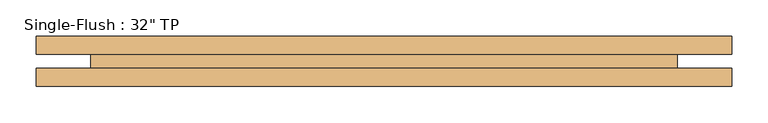
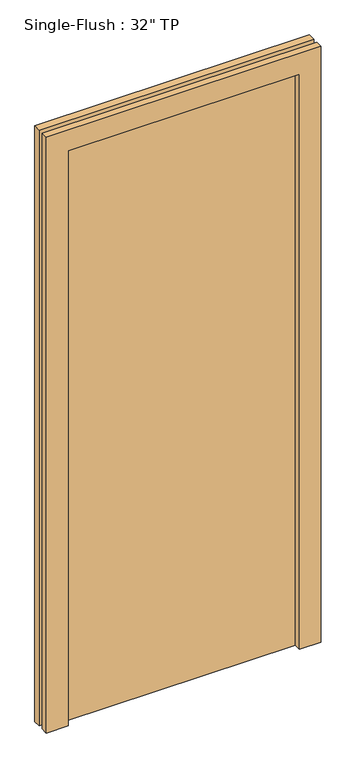
"""IFC4 building model written with IfcOpenShell, lengths in millimetres: door geometry."""

from ifc_helpers import new_model, si_unit, frame, origin, origin_with_axes, place, context, project, spatial, polyline, outline, extrude, source, transform, mapped, element, save


def door_1d070c31(model_context):
    return source(origin(), model_context, "Body", "SweptSolid", [
        extrude(outline(polyline([(2209.8, -482.6), (0.0, -482.6), (0.0, -406.4), (2133.6, -406.4), (2133.6, 406.4), (0.0, 406.4), (0.0, 482.6), (2209.8, 482.6), (2209.8, -482.6)])), frame((0.0, -34.925, 0.0), z_axis=(0.0, 1.0, 0.0), x_axis=(0.0, 0.0, 1.0)), (0.0, 0.0, 1.0), 25.4),
        extrude(outline(polyline([(2209.8, 482.6), (2209.8, -482.6), (0.0, -482.6), (0.0, -406.4), (2133.6, -406.4), (2133.6, 406.4), (0.0, 406.4), (0.0, 482.6), (2209.8, 482.6)])), frame((0.0, 9.525, 0.0), z_axis=(0.0, 1.0, 0.0), x_axis=(0.0, 0.0, 1.0)), (0.0, 0.0, 1.0), 25.4),
        extrude(outline(polyline([(406.4, 9.525), (406.4, -9.525), (-406.4, -9.525), (-406.4, 9.525), (406.4, 9.525)])), origin_with_axes(), (0.0, 0.0, 1.0), 2133.6),
    ])


if __name__ == "__main__":
    model = new_model("IFC4")
    model_context = context("Model", 3, world=origin())
    ifc_project = project(units=[si_unit("LENGTHUNIT", "METRE", prefix="MILLI")], contexts=[model_context])
    site = spatial("IfcSite", under=ifc_project)
    building = spatial("IfcBuilding", under=site)
    placement = place(None, origin())
    door_shape = door_1d070c31(model_context)
    element("IfcDoor", 1, ObjectType="Single-Flush : 32\" TP", at=placement, inside=building, context=model_context, shape_type="MappedRepresentation", body=[
        mapped(door_shape, transform((0.0, 0.0, 0.0), x_axis=(1.0, 0.0, 0.0), y_axis=(0.0, 1.0, 0.0), z_axis=(0.0, 0.0, 1.0))),
    ])
    save(model, "model.ifc")

# Revit data of these elements
# Type "Single-Flush : 32\" TP"
#   Type Mark = "58"
#   Construction Type Id = "MDOOR"
#   Assembly Code = "C1020"
#   Analytic Construction = "Metal"
#   Thickness = 0' - 0 3/4"
#   Heat Transfer Coefficient (U) = 3.7021 W/(m²·K)
#   Height = 7' - 0"
#   Trim Projection Ext = 0' - 1"
#   Trim Projection Int = 0' - 1"
#   Trim Width = 0' - 3"
#   Width = 2' - 8"
#   Door Material = Door - Panel
#   Frame Material = Door - Frame
#   Visual Light Transmittance = 0
#   Solar Heat Gain Coefficient = 0
#   Function = (empty or 0)
#   Wall Closure = (empty or 0)
# Element 1 (IfcDoor, "Single-Flush : 32\" TP")
#   Materials on its faces: "Door - Frame", "Door - Panel"
# Materials
#   "Door - Panel": class "Wood", colour RGB 210 159 95, transparency 0
#   "Door - Frame": class "Miscellaneous", colour RGB 118 70 51, transparency 0
